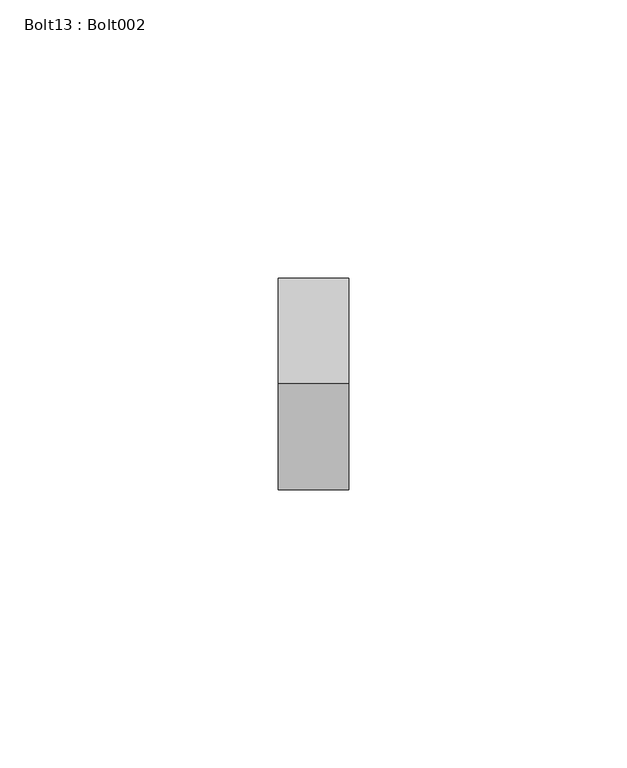
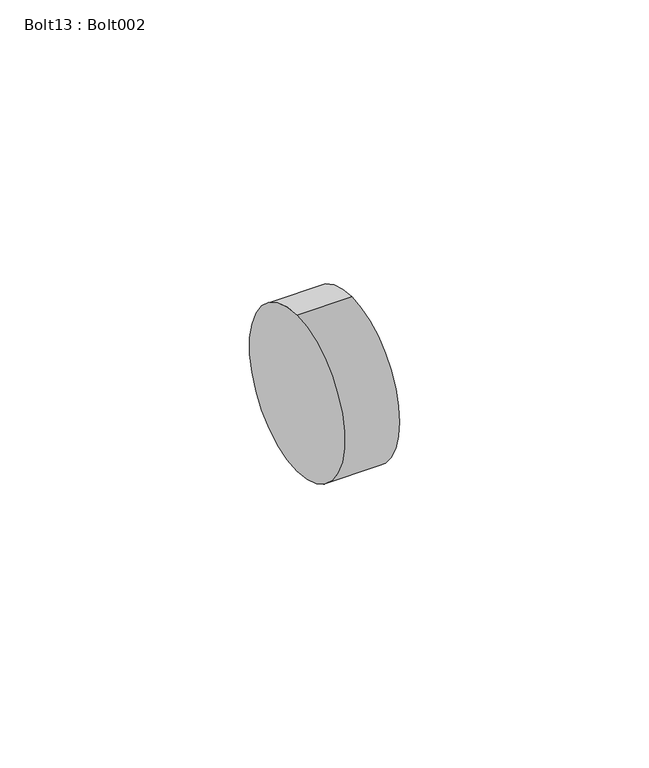
"""IFC4 building model written with IfcOpenShell, lengths in millimetres: proxy geometry, Bolt13 : Bolt002."""

from ifc_helpers import new_model, si_unit, point, frame, frame_2d, origin, place, context, project, spatial, circle_curve, trimmed, segment, composite_curve, outline, extrude, source, transform, mapped, element, save


def bolt13_bolt002_48e6a7b8(model_context):
    return source(origin(), model_context, "Body", "SweptSolid", [
        extrude(outline(composite_curve([segment(trimmed(circle_curve(frame_2d((1896.5882072, 40070.0545241)), 19.05), [point((1896.5882072, 40051.0045241))], [point((1896.5882072, 40089.1045241))], False, "CARTESIAN"), True, "CONTINUOUS"), segment(trimmed(circle_curve(frame_2d((1896.5882072, 40070.0545241)), 19.05), [point((1896.5882072, 40089.1045241))], [point((1896.5882072, 40051.0045241))], False, "CARTESIAN"), True, "CONTINUOUS")], self_intersect=False)), frame((10297.8384869, 0.0, 0.0), z_axis=(1.0, 0.0, 0.0), x_axis=(0.0, 1.0, 0.0)), (0.0, 0.0, 1.0), 12.7),
    ])


if __name__ == "__main__":
    model = new_model("IFC4")
    model_context = context("Model", 3, world=origin())
    ifc_project = project(units=[si_unit("LENGTHUNIT", "METRE", prefix="MILLI")], contexts=[model_context])
    site = spatial("IfcSite", under=ifc_project)
    building = spatial("IfcBuilding", under=site)
    placement = place(None, origin())
    bolt13_bolt002_shape = bolt13_bolt002_48e6a7b8(model_context)
    element("IfcBuildingElementProxy", 1, Name="Bolt13 : Bolt002", ObjectType="Bolt13 : Bolt002", at=placement, inside=building, context=model_context, shape_type="MappedRepresentation", body=[
        mapped(bolt13_bolt002_shape, transform((0.0, 0.0, 0.0), x_axis=(1.0, 0.0, 0.0), y_axis=(0.0, 1.0, 0.0), z_axis=(0.0, 0.0, 1.0))),
    ])
    save(model, "model.ifc")

# Revit data of these elements
# Type "Bolt13 : Bolt002"
#   NameOverride = "Bolt002"
# Element 1 (IfcBuildingElementProxy, "Bolt13 : Bolt002")
#   Materials on its faces: "TUBE STEEL STRINGER WELDED TO ANCHORED STEEL PLATE - SEE STRUCT DWGS"
# Materials
#   "TUBE STEEL STRINGER WELDED TO ANCHORED STEEL PLATE - SEE STRUCT DWGS": class "Unassigned", colour RGB 128 128 128, transparency 0, Cost = 0
